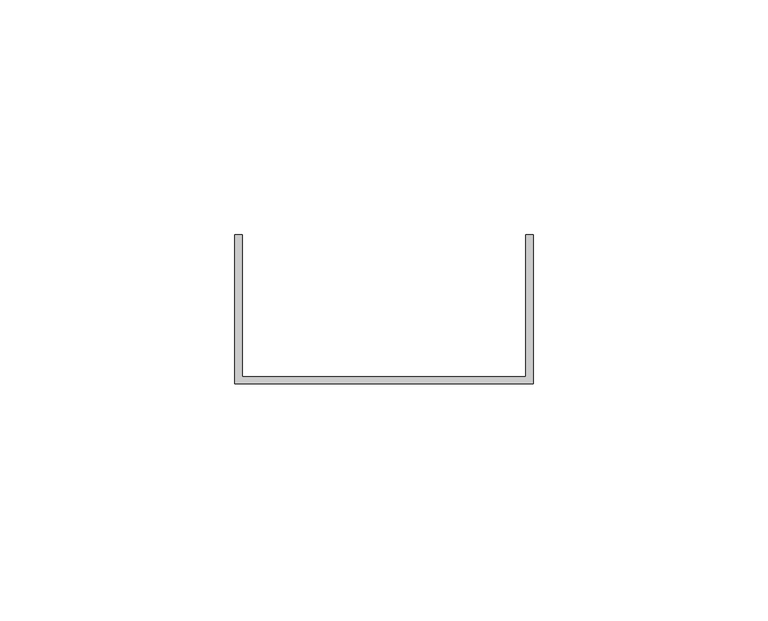
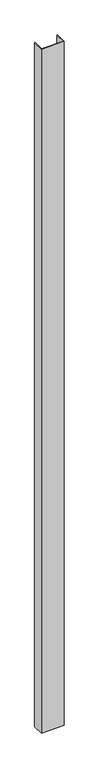
"""IFC4 building model written with IfcOpenShell, lengths in millimetres: proxy geometry, Generic Models 7:Generic Models 1:3:Generic Models 1:3 : Generic Models 7:Generic Models 1:305549:3:Generic Models 1:3:Generic Models 1:3 : Generic Models 7:Generic Models 1:305549:3 : Generic Models 7:Generic Models 1:3:Generic Models 1:3 : Generic Models 7:Generic Models 1:305549:301244:25 : Generic Models 7:Generic Models 1:3:Generic Models 1:3 : Generic Models 7:Generic Models 1:305549:3:Generic Models 1:3:Generic Models 1:3 : Generic Models 7:Generic Models 1:305549:3 : Generic Models 7:Generic Models 1:3:Generic Models 1:3 : Generic Models 7:Generic Models 1:305549:301244:308848."""

import ifcopenshell
import ifcopenshell.guid

model = None  # the IFC model being written
_history = None  # IfcOwnerHistory: only IFC2X3 demands one
_inside = {}  # id of a spatial element -> (the spatial element, [elements in it])
_under = {}  # id of a project, library or spatial element -> (it, [spatial elements below it])
_declared = {}  # id of a project -> (the project, [libraries it declares])
_typed = {}  # id of a type object -> (the type object, [elements of that type])
_made_of = {}  # id of a material, layer set ... -> (it, [elements and type objects made of it])


def new_model(schema):
    """Start an empty IFC model of exactly this schema.

    Asked for "IFC4X3", IfcOpenShell would pick the latest addendum, in which some entities
    have other attributes; the version numbers below select the first issue.
    IFC2X3 requires an IfcOwnerHistory on every rooted entity: one is made here for all.
    """
    global model, _history
    if schema == "IFC4X3":
        model = ifcopenshell.file(schema_version=(4, 3, 0, 0))
    else:
        model = ifcopenshell.file(schema=schema)
    _inside.clear()
    _under.clear()
    _declared.clear()
    _typed.clear()
    _made_of.clear()
    _history = None
    if model.schema == "IFC2X3":
        org = make("IfcOrganization", Name="unknown")
        user = make(
            "IfcPersonAndOrganization",
            ThePerson=make("IfcPerson", FamilyName="unknown"),
            TheOrganization=org,
        )
        app = make(
            "IfcApplication",
            ApplicationDeveloper=org,
            Version="unknown",
            ApplicationFullName="unknown",
            ApplicationIdentifier="unknown",
        )
        _history = make(
            "IfcOwnerHistory",
            OwningUser=user,
            OwningApplication=app,
            ChangeAction="ADDED",
            CreationDate=0,
        )
    return model


def make(cls, **values):
    """One entity of the class cls with the attributes given. An attribute that is None is left unset."""
    return model.create_entity(
        cls, **{name: value for name, value in values.items() if value is not None}
    )


def rooted(cls, **values):
    """An entity with a GlobalId (a new one), such as an element, a storey or a relation."""
    return make(cls, GlobalId=ifcopenshell.guid.new(), OwnerHistory=_history, **values)


def si_unit(unit_type, name, prefix=None):
    """IfcSIUnit, for example si_unit("LENGTHUNIT", "METRE", prefix="MILLI")."""
    return make("IfcSIUnit", UnitType=unit_type, Prefix=prefix, Name=name)


def assignment(units):
    """IfcUnitAssignment: the units of a project."""
    return None if units is None else make("IfcUnitAssignment", Units=units)


def point(xyz):
    """IfcCartesianPoint."""
    return None if xyz is None else make("IfcCartesianPoint", Coordinates=xyz)


def direction(xyz):
    """IfcDirection."""
    return None if xyz is None else make("IfcDirection", DirectionRatios=xyz)


def frame(location, z_axis=None, x_axis=None):
    """IfcAxis2Placement3D, a coordinate frame: its origin and axes. An axis left out is left unset."""
    return make(
        "IfcAxis2Placement3D",
        Location=point(location),
        Axis=direction(z_axis),
        RefDirection=direction(x_axis),
    )


def origin():
    """The frame at (0, 0, 0) with its axes left unset."""
    return frame((0.0, 0.0, 0.0))


def place(relative_to, where):
    """IfcLocalPlacement: puts the frame where relative to a parent placement (None: the world)."""
    return make(
        "IfcLocalPlacement", PlacementRelTo=relative_to, RelativePlacement=where
    )


def context(
    kind, dimensions, precision=None, world=None, true_north=None, identifier=None
):
    """IfcGeometricRepresentationContext, for example the 3D "Model" context."""
    return make(
        "IfcGeometricRepresentationContext",
        ContextIdentifier=identifier,
        ContextType=kind,
        CoordinateSpaceDimension=dimensions,
        Precision=precision,
        WorldCoordinateSystem=world,
        TrueNorth=true_north,
    )


def project(units=None, contexts=None):
    """IfcProject with its units and contexts."""
    return rooted(
        "IfcProject",
        Name="project",
        RepresentationContexts=contexts,
        UnitsInContext=assignment(units),
    )


def spatial(cls, under=None, at=None, **own):
    """A site, building, storey or space (cls), placed at a placement, below another one or the project."""
    s = rooted(cls, ObjectPlacement=at, **own)
    if under is not None:
        _under.setdefault(under.id(), (under, []))[1].append(s)
    return s


def polyline(points):
    """IfcPolyline through the points."""
    return make("IfcPolyline", Points=[point(p) for p in points])


def outline(outer, holes=None, kind="AREA"):
    """IfcArbitraryClosedProfileDef: a profile drawn as a closed curve; with holes, ...WithVoids."""
    if holes is None:
        return make("IfcArbitraryClosedProfileDef", ProfileType=kind, OuterCurve=outer)
    return make(
        "IfcArbitraryProfileDefWithVoids",
        ProfileType=kind,
        OuterCurve=outer,
        InnerCurves=holes,
    )


def extrude(swept, where, along, depth):
    """IfcExtrudedAreaSolid: the profile swept, set in the frame where, extruded along a direction by depth."""
    return make(
        "IfcExtrudedAreaSolid",
        SweptArea=swept,
        Position=where,
        ExtrudedDirection=direction(along),
        Depth=depth,
    )


def shape(context_of_items, identifier, shape_type, items):
    """IfcShapeRepresentation: the items that make up one representation, for example the "Body"."""
    return make(
        "IfcShapeRepresentation",
        ContextOfItems=context_of_items,
        RepresentationIdentifier=identifier,
        RepresentationType=shape_type,
        Items=items,
    )


def source(mapping_origin, context_of_items, identifier, shape_type, items):
    """IfcRepresentationMap: a shape defined once, which mapped items show again and again."""
    return make(
        "IfcRepresentationMap",
        MappingOrigin=mapping_origin,
        MappedRepresentation=shape(context_of_items, identifier, shape_type, items),
    )


def transform(
    local_origin,
    x_axis=None,
    y_axis=None,
    z_axis=None,
    scale=None,
    scale2=None,
    scale3=None,
    uniform=True,
):
    """IfcCartesianTransformationOperator3D, or its non-uniform kind. x_axis, y_axis, z_axis: its Axis1, 2, 3."""
    if uniform:
        return make(
            "IfcCartesianTransformationOperator3D",
            Axis1=direction(x_axis),
            Axis2=direction(y_axis),
            LocalOrigin=point(local_origin),
            Scale=scale,
            Axis3=direction(z_axis),
        )
    return make(
        "IfcCartesianTransformationOperator3DnonUniform",
        Axis1=direction(x_axis),
        Axis2=direction(y_axis),
        LocalOrigin=point(local_origin),
        Scale=scale,
        Axis3=direction(z_axis),
        Scale2=scale2,
        Scale3=scale3,
    )


def mapped(mapping_source, mapping_target):
    """IfcMappedItem: shows the shape of a source again, moved by a transform."""
    return make(
        "IfcMappedItem", MappingSource=mapping_source, MappingTarget=mapping_target
    )


def made_of(thing, what):
    """Note that an element or type object is made of a material, layer set ...; save() writes the relation."""
    if what is not None:
        _made_of.setdefault(what.id(), (what, []))[1].append(thing)
    return thing


def element(
    cls,
    number,
    at=None,
    inside=None,
    cuts=None,
    type_object=None,
    material=None,
    context=None,
    identifier="Body",
    shape_type=None,
    held_by="IfcProductDefinitionShape",
    body=None,
    shapes=None,
    **own,
):
    """One element of the class cls, such as IfcWall. Its Tag is "e" and its number.

    at: its placement. inside: the storey or other place that contains it. cuts: it is an
    opening in that element (IfcRelVoidsElement). A single representation is given by context,
    identifier, shape_type and body (its items); several are given by shapes. held_by: the class
    of the entity that holds the representations. save() writes the other relations.
    """
    e = rooted(cls, Tag="e%d" % number, ObjectPlacement=at, **own)
    if body is not None:
        shapes = [shape(context, identifier, shape_type, body)]
    if shapes is not None:
        e.Representation = make(held_by, Representations=shapes)
    if inside is not None:
        _inside.setdefault(inside.id(), (inside, []))[1].append(e)
    if cuts is not None:
        rooted(
            "IfcRelVoidsElement", RelatingBuildingElement=cuts, RelatedOpeningElement=e
        )
    if type_object is not None:
        _typed.setdefault(type_object.id(), (type_object, []))[1].append(e)
    return made_of(e, material)


def aggregate(whole, parts):
    """IfcRelAggregates: a whole, such as a stair, and the parts it consists of."""
    return rooted("IfcRelAggregates", RelatingObject=whole, RelatedObjects=parts)


def save(model, path):
    """Write the relations noted so far, then the file.

    IfcRelAggregates (storeys below a building ...), IfcRelContainedInSpatialStructure (elements
    in a storey), IfcRelDefinesByType, IfcRelAssociatesMaterial and IfcRelDeclares: one each for
    every whole, place, type object, material and project.
    """
    for whole, parts in _under.values():
        aggregate(whole, parts)
    for where, things in _inside.values():
        rooted(
            "IfcRelContainedInSpatialStructure",
            RelatedElements=things,
            RelatingStructure=where,
        )
    for kind, things in _typed.values():
        rooted("IfcRelDefinesByType", RelatedObjects=things, RelatingType=kind)
    for what, things in _made_of.values():
        rooted("IfcRelAssociatesMaterial", RelatedObjects=things, RelatingMaterial=what)
    for by, libraries in _declared.values():
        rooted("IfcRelDeclares", RelatingContext=by, RelatedDefinitions=libraries)
    model.write(path)


def generic_models_c012fa72(model_context):
    return source(origin(), model_context, "Body", "SweptSolid", [
        extrude(outline(polyline([(560352.9617239, -579000.6913841), (560289.4617239, -579000.6913841), (560289.4617239, -578968.9413841), (560291.0492239, -578968.9413841), (560291.0492239, -578999.1038841), (560351.3742239, -578999.1038841), (560351.3742239, -578968.9413841), (560352.9617239, -578968.9413841), (560352.9617239, -579000.6913841)])), frame((0.0, 0.0, 4133.81326), z_axis=(0.0, 0.0, 1.0), x_axis=(1.0, 0.0, 0.0)), (0.0, 0.0, 1.0), 2000.28674),
    ])


if __name__ == "__main__":
    model = new_model("IFC4")
    model_context = context("Model", 3, world=origin())
    ifc_project = project(units=[si_unit("LENGTHUNIT", "METRE", prefix="MILLI")], contexts=[model_context])
    site = spatial("IfcSite", under=ifc_project)
    building = spatial("IfcBuilding", under=site)
    placement = place(None, origin())
    generic_models_shape = generic_models_c012fa72(model_context)
    element("IfcBuildingElementProxy", 1, Name="Generic Models 7:Generic Models 1:3:Generic Models 1:3 : Generic Models 7:Generic Models 1:305549:3:Generic Models 1:3:Generic Models 1:3 : Generic Models 7:Generic Models 1:305549:3 : Generic Models 7:Generic Models 1:3:Generic Models 1:3 : Generic Models 7:Generic Models 1:305549:301244:25 : Generic Models 7:Generic Models 1:3:Generic Models 1:3 : Generic Models 7:Generic Models 1:305549:3:Generic Models 1:3:Generic Models 1:3 : Generic Models 7:Generic Models 1:305549:3 : Generic Models 7:Generic Models 1:3:Generic Models 1:3 : Generic Models 7:Generic Models 1:305549:301244:308848", ObjectType="Generic Models 7:Generic Models 1:3:Generic Models 1:3 : Generic Models 7:Generic Models 1:305549:3:Generic Models 1:3:Generic Models 1:3 : Generic Models 7:Generic Models 1:305549:3 : Generic Models 7:Generic Models 1:3:Generic Models 1:3 : Generic Models 7:Generic Models 1:305549:301244:25 : Generic Models 7:Generic Models 1:3:Generic Models 1:3 : Generic Models 7:Generic Models 1:305549:3:Generic Models 1:3:Generic Models 1:3 : Generic Models 7:Generic Models 1:305549:3 : Generic Models 7:Generic Models 1:3:Generic Models 1:3 : Generic Models 7:Generic Models 1:305549:301244:308848", at=placement, inside=building, context=model_context, shape_type="MappedRepresentation", body=[
        mapped(generic_models_shape, transform((0.0, 0.0, 0.0), x_axis=(1.0, 0.0, 0.0), y_axis=(0.0, 1.0, 0.0), z_axis=(0.0, 0.0, 1.0))),
    ])
    save(model, "model.ifc")

# Revit data of these elements
# Type "Generic Models 7:Generic Models 1:3:Generic Models 1:3 : Generic Models 7:Generic Models 1:305549:3:Generic Models 1:3:Generic Models 1:3 : Generic Models 7:Generic Models 1:305549:3 : Generic Models 7:Generic Models 1:3:Generic Models 1:3 : Generic Models 7:Generic Models 1:305549:301244:25 : Generic Models 7:Generic Models 1:3:Generic Models 1:3 : Generic Models 7:Generic Models 1:305549:3:Generic Models 1:3:Generic Models 1:3 : Generic Models 7:Generic Models 1:305549:3 : Generic Models 7:Generic Models 1:3:Generic Models 1:3 : Generic Models 7:Generic Models 1:305549:301244:308848"
#   NameOverride = "Generic Models 7:Generic Models 1:3:Generic Models 1:3 : Generic Models 7:Generic Models 1:305549:3:Generic Models 1:3:Generic Models 1:3 : Generic Models 7:Generic Models 1:305549:3 : Generic Models 7:Generic Models 1:3:Generic Models 1:3 : Generic Models 7:Generic Models 1:305549:301244:308848"
#   ObjectTypeOverride = "Generic Models 1:3:Generic Models 1:3 : Generic Models 7:Generic Models 1:305549:3 : Generic Models 7:Generic Models 1:3:Generic Models 1:3 : Generic Models 7:Generic Models 1:305549:301244"
#   Reference = "Generic Models 1"
#   Tag = "308848"
# Element 1 (IfcBuildingElementProxy, "Generic Models 7:Generic Models 1:3:Generic Models 1:3 : Generic Models 7:Generic Models 1:305549:3:Generic Models 1:3:Generic Models 1:3 : Generic Models 7:Generic Models 1:305549:3 : Generic Models 7:Generic Models 1:3:Generic Models 1:3 : Generic Models 7:Generic Models 1:305549:301244:25 : Generic Models 7:Generic Models 1:3:Generic Models 1:3 : Generic Models 7:Generic Models 1:305549:3:Generic Models 1:3:Generic Models 1:3 : Generic Models 7:Generic Models 1:305549:3 : Generic Models 7:Generic Models 1:3:Generic Models 1:3 : Generic Models 7:Generic Models 1:305549:301244:308848")
#   Materials on its faces: "GALVANIZED U-CHANNEL (250T125-33)"
# Materials
#   "GALVANIZED U-CHANNEL (250T125-33)": class "Unassigned", colour RGB 202 201 200, transparency 0, Keynote = "M05451300.02", Cost = 0
